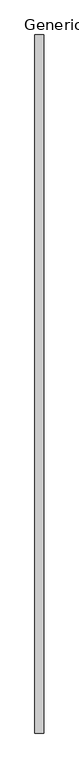
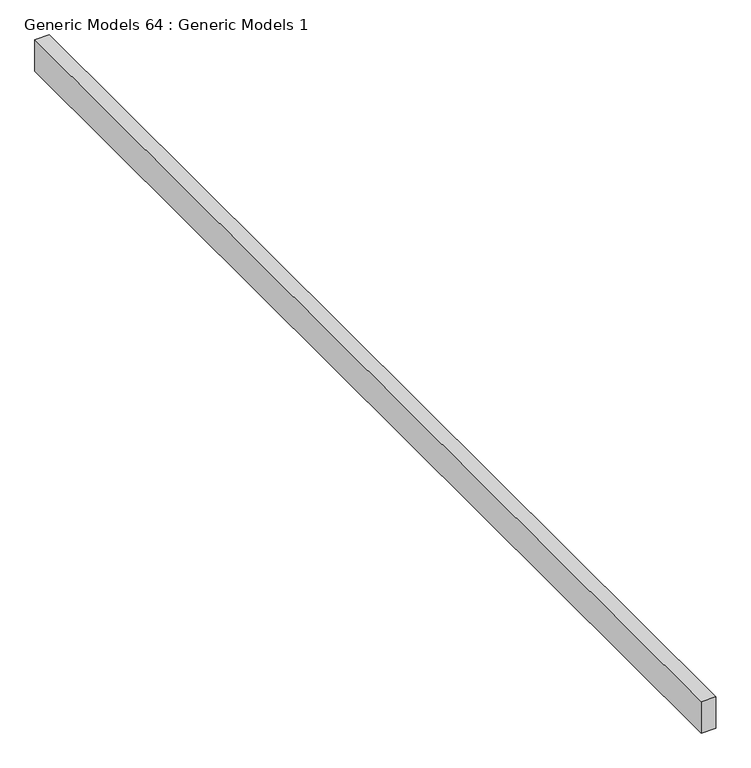
"""IFC4 building model written with IfcOpenShell, lengths in millimetres: proxy geometry, Generic Models 64 : Generic Models 1."""

from ifc_helpers import new_model, si_unit, frame, origin, place, context, project, spatial, polyline, outline, extrude, source, transform, mapped, element, save


def generic_models_64_generic_models_1_127614b5(model_context):
    return source(origin(), model_context, "Body", "SweptSolid", [
        extrude(outline(polyline([(-9436.2736296, 7054.2769662), (-9258.4736296, 7054.2769662), (-9258.4736296, -7068.1230338), (-9436.2736296, -7068.1230338), (-9436.2736296, 7054.2769662)])), frame((0.0, 0.0, 126345.696), z_axis=(0.0, 0.0, 1.0), x_axis=(1.0, 0.0, 0.0)), (0.0, 0.0, 1.0), 406.4),
    ])


if __name__ == "__main__":
    model = new_model("IFC4")
    model_context = context("Model", 3, world=origin())
    ifc_project = project(units=[si_unit("LENGTHUNIT", "METRE", prefix="MILLI")], contexts=[model_context])
    site = spatial("IfcSite", under=ifc_project)
    building = spatial("IfcBuilding", under=site)
    placement = place(None, origin())
    generic_models_64_generic_models_1_shape = generic_models_64_generic_models_1_127614b5(model_context)
    element("IfcBuildingElementProxy", 1, Name="Generic Models 64 : Generic Models 1", ObjectType="Generic Models 64 : Generic Models 1", at=placement, inside=building, context=model_context, shape_type="MappedRepresentation", body=[
        mapped(generic_models_64_generic_models_1_shape, transform((0.0, 0.0, 0.0), x_axis=(1.0, 0.0, 0.0), y_axis=(0.0, 1.0, 0.0), z_axis=(0.0, 0.0, 1.0))),
    ])
    save(model, "model.ifc")

# Revit data of these elements
# Element 1 (IfcBuildingElementProxy, "Generic Models 64 : Generic Models 1")
#   Materials on its faces: "_STRUCTURAL MEMBER (SEE STRUCT. DWGS)"
# Materials
#   "_STRUCTURAL MEMBER (SEE STRUCT. DWGS)": class "Generic", colour RGB 209 182 141, transparency 0, Cost = 0
